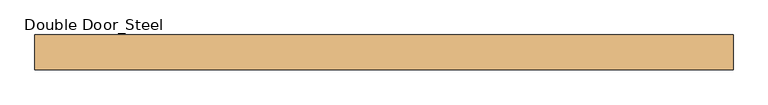
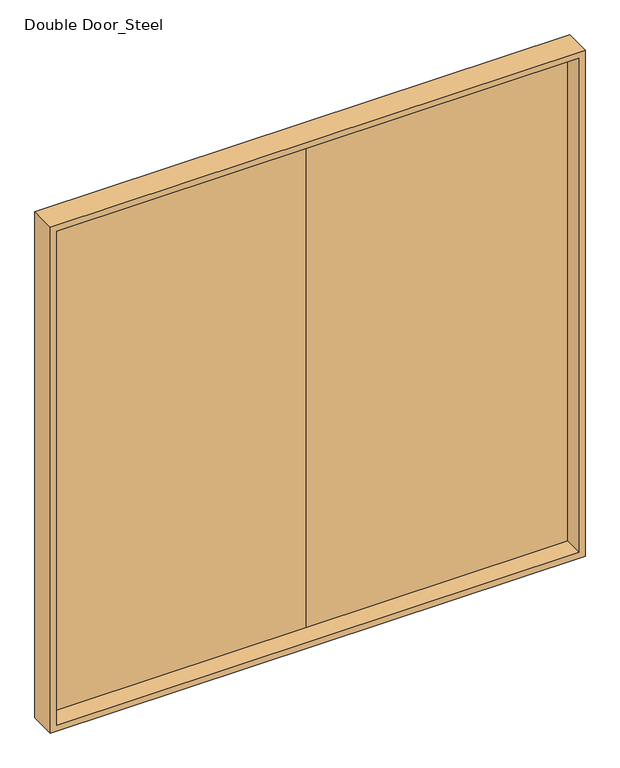
"""IFC4 building model written with IfcOpenShell, lengths in millimetres: door geometry, Double Door_Steel : H_DR_AR_B12_Double Door_Steel_W3000xH3000."""

from ifc_helpers import new_model, si_unit, frame, origin, place, context, project, spatial, polyline, outline, extrude, faceted_brep, source, transform, mapped, element, save


def double_door_steel_0432cfbf(model_context):
    return source(origin(), model_context, "Body", "SolidModel", [
        extrude(outline(polyline([(1480.0, 35.0), (0.0, 35.0), (0.0, 75.0), (1480.0, 75.0), (1480.0, 35.0)])), frame((0.0, 0.0, 20.0), z_axis=(0.0, 0.0, 1.0), x_axis=(1.0, 0.0, 0.0)), (0.0, 0.0, 1.0), 2960.0),
        extrude(outline(polyline([(0.0, 35.0), (-1480.0, 35.0), (-1480.0, 75.0), (0.0, 75.0), (0.0, 35.0)])), frame((0.0, 0.0, 20.0), z_axis=(0.0, 0.0, 1.0), x_axis=(1.0, 0.0, 0.0)), (0.0, 0.0, 1.0), 2960.0),
        faceted_brep([(1500.0, -75.0, 3000.0), (1500.0, 75.0, 3000.0), (-1500.0, 75.0, 3000.0), (-1500.0, -75.0, 3000.0), (1465.0, 35.0, 2965.0), (1465.0, -75.0, 2965.0), (-1465.0, -75.0, 2965.0), (-1465.0, 35.0, 2965.0), (1480.0, 75.0, 2980.0), (1480.0, 35.0, 2980.0), (-1480.0, 35.0, 2980.0), (-1480.0, 75.0, 2980.0), (-1500.0, 75.0, 0.0), (-1500.0, -75.0, 0.0), (-1465.0, -75.0, 35.0), (-1465.0, 35.0, 35.0), (-1480.0, 35.0, 20.0), (-1480.0, 75.0, 20.0), (1500.0, 75.0, 0.0), (1480.0, 75.0, 20.0), (1500.0, -75.0, 0.0), (1465.0, -75.0, 35.0), (1465.0, 35.0, 35.0), (1480.0, 35.0, 20.0)], [[[0, 1, 2, 3]], [[4, 5, 6, 7]], [[8, 9, 10, 11]], [[3, 2, 12, 13]], [[7, 6, 14, 15]], [[11, 10, 16, 17]], [[18, 12, 2, 1], [8, 11, 17, 19]], [[13, 12, 18, 20]], [[0, 3, 13, 20], [21, 14, 6, 5]], [[15, 14, 21, 22]], [[23, 16, 10, 9], [4, 7, 15, 22]], [[17, 16, 23, 19]], [[20, 18, 1, 0]], [[22, 21, 5, 4]], [[19, 23, 9, 8]]]),
    ])


if __name__ == "__main__":
    model = new_model("IFC4")
    model_context = context("Model", 3, world=origin())
    ifc_project = project(units=[si_unit("LENGTHUNIT", "METRE", prefix="MILLI")], contexts=[model_context])
    site = spatial("IfcSite", under=ifc_project)
    building = spatial("IfcBuilding", under=site)
    placement = place(None, origin())
    double_door_steel_shape = double_door_steel_0432cfbf(model_context)
    element("IfcDoor", 1, ObjectType="Double Door_Steel : H_DR_AR_B12_Double Door_Steel_W3000xH3000", at=placement, inside=building, context=model_context, shape_type="MappedRepresentation", body=[
        mapped(double_door_steel_shape, transform((0.0, 0.0, 0.0), x_axis=(1.0, 0.0, 0.0), y_axis=(0.0, 1.0, 0.0), z_axis=(0.0, 0.0, 1.0))),
    ])
    save(model, "model.ifc")

# Revit data of these elements
# Type "Double Door_Steel : H_DR_AR_B12_Double Door_Steel_W3000xH3000"
#   Type Mark = "430"
#   프레임 = ""
#   철물 = ""
#   유리/마감 = ""
#   위치/개소 = ""
#   부호 = "1/SD"
#   문번호 = ""
#   문기호 = "SD"
#   Analytic Construction = "<None>"
#   Height = 3000 mm
#   Width = 3000 mm
#   Define Thermal Properties by = 1
#   문 틀 = none
#   문 = none
#   Function = (empty or 0)
#   Assembly Code = ""
#   Wall Closure = (empty or 0)
